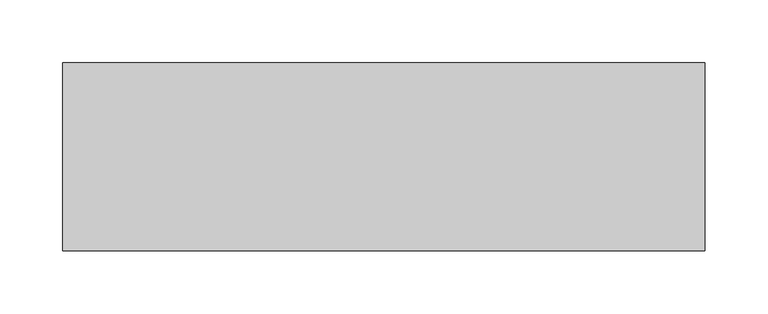
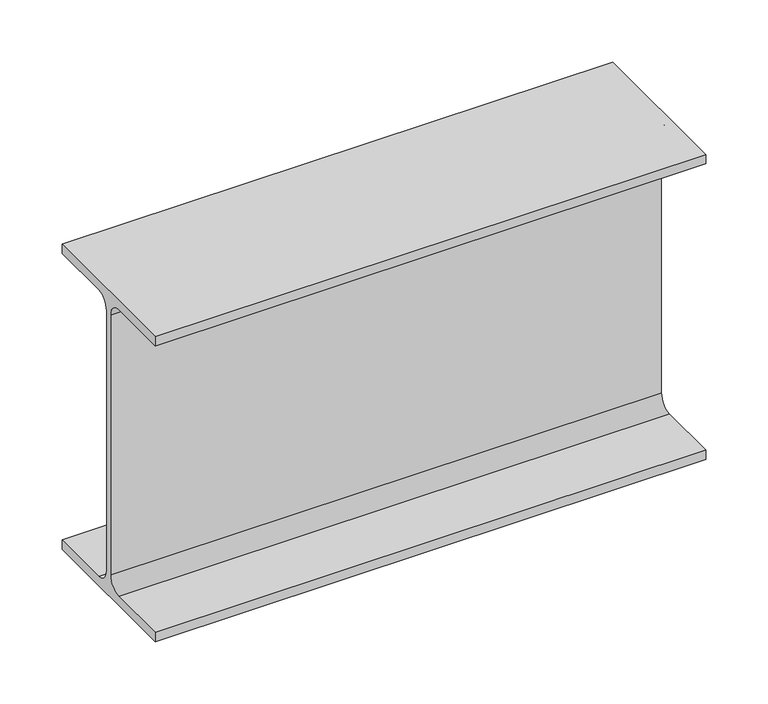
"""IFC4 building model written with IfcOpenShell, lengths in millimetres: beam geometry, 0912_Steel Framing_H-KSD3502 : H_SB_ASB_H-300x150x6.5x9."""

from ifc_helpers import new_model, si_unit, point, frame, frame_2d, origin, place, context, project, spatial, polyline, circle_curve, trimmed, segment, composite_curve, outline, extrude, source, transform, mapped, element, save


def beam_eaea1fdd(model_context):
    return source(origin(), model_context, "Body", "SweptSolid", [
        extrude(outline(composite_curve([segment(polyline([(75.0, -141.0), (75.0, -150.0), (-75.0, -150.0), (-75.0, -141.0), (-16.25, -141.0)]), True, "CONTINUOUS"), segment(trimmed(circle_curve(frame_2d((-16.25, -128.0)), 13.0), [point((-16.25, -141.0))], [point((-3.25, -128.0))], True, "CARTESIAN"), True, "CONTINUOUS"), segment(polyline([(-3.25, -128.0), (-3.25, 128.0)]), True, "CONTINUOUS"), segment(trimmed(circle_curve(frame_2d((-16.25, 128.0)), 13.0), [point((-3.25, 128.0))], [point((-16.25, 141.0))], True, "CARTESIAN"), True, "CONTINUOUS"), segment(polyline([(-16.25, 141.0), (-75.0, 141.0), (-75.0, 150.0), (75.0, 150.0), (75.0, 141.0), (16.25, 141.0)]), True, "CONTINUOUS"), segment(trimmed(circle_curve(frame_2d((16.25, 128.0)), 13.0), [point((16.25, 141.0))], [point((3.25, 128.0))], True, "CARTESIAN"), True, "CONTINUOUS"), segment(polyline([(3.25, 128.0), (3.25, -128.0)]), True, "CONTINUOUS"), segment(trimmed(circle_curve(frame_2d((16.25, -128.0)), 13.0), [point((3.25, -128.0))], [point((16.25, -141.0))], True, "CARTESIAN"), True, "CONTINUOUS"), segment(polyline([(16.25, -141.0), (75.0, -141.0)]), True, "CONTINUOUS")], self_intersect=False)), frame((-300.0, 0.0, 0.0), z_axis=(1.0, 0.0, 0.0), x_axis=(0.0, 1.0, 0.0)), (0.0, 0.0, 1.0), 512.3),
    ])


if __name__ == "__main__":
    model = new_model("IFC4")
    model_context = context("Model", 3, world=origin())
    ifc_project = project(units=[si_unit("LENGTHUNIT", "METRE", prefix="MILLI")], contexts=[model_context])
    site = spatial("IfcSite", under=ifc_project)
    building = spatial("IfcBuilding", under=site)
    placement = place(None, origin())
    beam_shape = beam_eaea1fdd(model_context)
    element("IfcBeam", 1, ObjectType="0912_Steel Framing_H-KSD3502 : H_SB_ASB_H-300x150x6.5x9", at=placement, inside=building, context=model_context, shape_type="MappedRepresentation", body=[
        mapped(beam_shape, transform((0.0, 0.0, 0.0), x_axis=(1.0, 0.0, 0.0), y_axis=(0.0, 1.0, 0.0), z_axis=(0.0, 0.0, 1.0))),
    ])
    save(model, "model.ifc")

# Revit data of these elements
# Type "0912_Steel Framing_H-KSD3502 : H_SB_ASB_H-300x150x6.5x9"
#   H_WM Code_1 = "S01AA002-00001 | Main Steel Structure Fabrication Work | Shelter/Building | Medium Steel - Standard (90KG/M>Weight≥30KG/M) | Material: (   )"
#   H_WM Code_2 = "S03AA028-00001 | Main Steel Structure Erection Work | Shelter/Building | Medium Steel (90KG/M>Weight≥30KG/M) | Material: (   )"
#   H_WM Code_3 = "S01AA010-00001 | Main Steel Structure Fabrication Work | Shelter/Building | Steel Painting/Coating | for Non-Fireproofed Steel Surface, Surface Preparation, Primer, Second & Final Coat | Material: (   )"
#   H_Q'ty Cal Type Tag = "SB-Q2"
#   Width = 15.0 cm
#   Web Thickness = 0.65 cm
#   Web Fillet = 1.3 cm
#   Warping Constant = 107000.0 cm⁶
#   W = 0
#   Torsional Moment of Inertia = 9.9539 cm⁴
#   Section Area = 46.78 cm²
#   Plastic Modulus weak axis = 105.0 cm³
#   Plastic Modulus strong axis = 542.0 cm³
#   Perimeter = 1.17 m²/m
#   Nominal Weight = 36.70 kgf/m
#   Moment of Inertia weak axis = 508.00 cm⁴
#   Moment of Inertia strong axis = 7210.00 cm⁴
#   Height = 30.0 cm
#   Flange Thickness = 0.9 cm
#   Elastic Modulus weak axis = 67.7 cm³
#   Elastic Modulus strong axis = 481.0 cm³
#   Centroid Vertical = 15.0 cm
#   Centroid Horizontal = 7.5 cm
#   Ix = 72100000
#   Length [instance default] = 1.5240 m
#   Zx = 542000
#   b = 0.1500 m
#   h = 0.3000 m
#   r = 0.0130 m
#   s = 0.0065 m
#   t = 0.0090 m
#   A = 0.004678 m²
#   Structural Material [instance default] = Steel, 45-345
#   Assembly Code = ""
# Element 1 (IfcBeam, "0912_Steel Framing_H-KSD3502 : H_SB_ASB_H-300x150x6.5x9")
#   Structural Material = none
# Materials
#   "Steel, 45-345": class "Metal", colour RGB 189 187 185, transparency 0, Description = "Steel 345 MPa", Cost = 0
